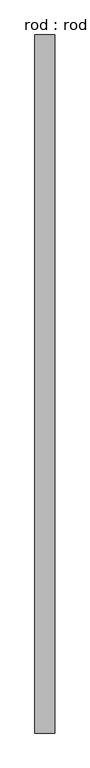
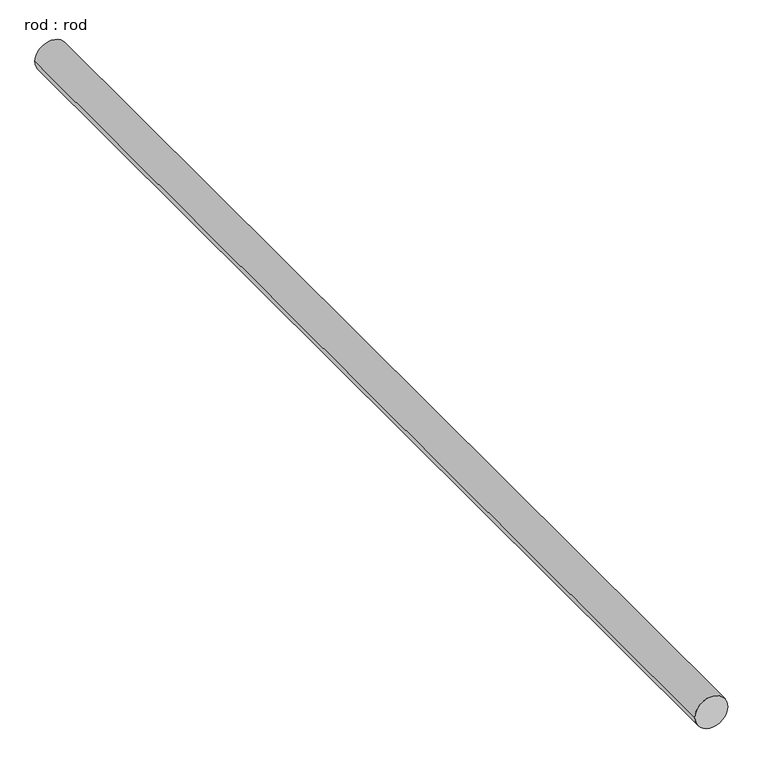
"""IFC4 building model written with IfcOpenShell, lengths in millimetres: proxy geometry, rod : rod."""

from ifc_helpers import new_model, si_unit, point, frame, frame_2d, origin, place, context, project, spatial, circle_curve, trimmed, segment, composite_curve, outline, extrude, source, transform, mapped, element, save


def rod_rod_3b4bddfe(model_context):
    return source(origin(), model_context, "Body", "SweptSolid", [
        extrude(outline(composite_curve([segment(trimmed(circle_curve(frame_2d((0.0108462, 0.0)), 200.0), [point((0.0108462, 200.0))], [point((0.0108462, -200.0))], False, "CARTESIAN"), True, "CONTINUOUS"), segment(trimmed(circle_curve(frame_2d((0.0108462, 0.0)), 200.0), [point((0.0108462, -200.0))], [point((0.0108462, 200.0))], False, "CARTESIAN"), True, "CONTINUOUS")], self_intersect=False)), frame((0.0, -2858.1642418, 0.0), z_axis=(0.0, 1.0, 0.0), x_axis=(0.0, 0.0, 1.0)), (0.0, 0.0, 1.0), 13901.7857143),
    ])


if __name__ == "__main__":
    model = new_model("IFC4")
    model_context = context("Model", 3, world=origin())
    ifc_project = project(units=[si_unit("LENGTHUNIT", "METRE", prefix="MILLI")], contexts=[model_context])
    site = spatial("IfcSite", under=ifc_project)
    building = spatial("IfcBuilding", under=site)
    placement = place(None, origin())
    rod_rod_shape = rod_rod_3b4bddfe(model_context)
    element("IfcBuildingElementProxy", 1, Name="rod : rod", ObjectType="rod : rod", at=placement, inside=building, context=model_context, shape_type="MappedRepresentation", body=[
        mapped(rod_rod_shape, transform((0.0, 0.0, 0.0), x_axis=(1.0, 0.0, 0.0), y_axis=(0.0, 1.0, 0.0), z_axis=(0.0, 0.0, 1.0))),
    ])
    save(model, "model.ifc")

# Revit data of these elements
# Type "rod : rod"
#   Default Elevation = 0
